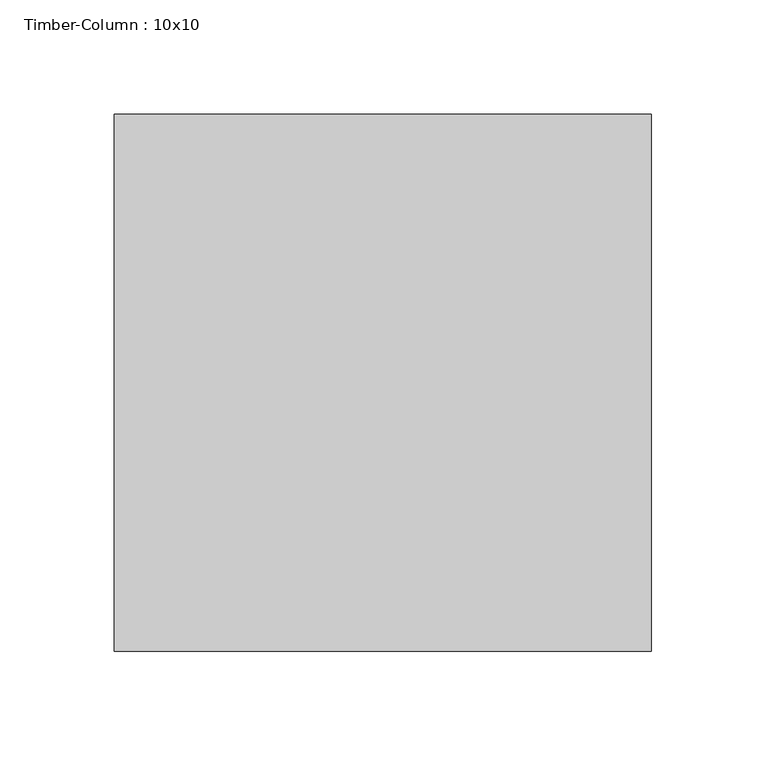
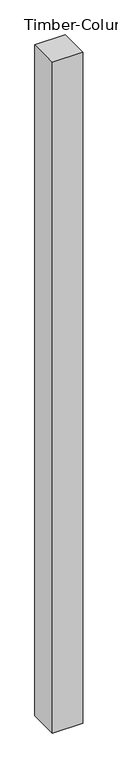
"""IFC4 building model written with IfcOpenShell, lengths in millimetres: column geometry, Timber-Column : 10x10."""

from ifc_helpers import new_model, si_unit, origin, origin_with_axes, place, context, project, spatial, polyline, outline, extrude, source, transform, mapped, element, save


def timber_column_10x10_5c3dec59(model_context):
    return source(origin(), model_context, "Body", "SweptSolid", [
        extrude(outline(polyline([(117.475, 117.475), (117.475, -117.475), (-117.475, -117.475), (-117.475, 117.475), (117.475, 117.475)])), origin_with_axes(), (0.0, 0.0, 1.0), 5486.4),
    ])


if __name__ == "__main__":
    model = new_model("IFC4")
    model_context = context("Model", 3, world=origin())
    ifc_project = project(units=[si_unit("LENGTHUNIT", "METRE", prefix="MILLI")], contexts=[model_context])
    site = spatial("IfcSite", under=ifc_project)
    building = spatial("IfcBuilding", under=site)
    placement = place(None, origin())
    timber_column_10x10_shape = timber_column_10x10_5c3dec59(model_context)
    element("IfcColumn", 1, ObjectType="Timber-Column : 10x10", at=placement, inside=building, context=model_context, shape_type="MappedRepresentation", body=[
        mapped(timber_column_10x10_shape, transform((0.0, 0.0, 0.0), x_axis=(1.0, 0.0, 0.0), y_axis=(0.0, 1.0, 0.0), z_axis=(0.0, 0.0, 1.0))),
    ])
    save(model, "model.ifc")

# Revit data of these elements
# Type "Timber-Column : 10x10"
#   Assembly Code = "B10"
#   A = 0.210069 SF
#   b = 0' - 9 1/4"
#   d = 0' - 9 1/4"
#   Structural Material = (4) CHARRED SISTERED 2X10s AT BEAM
# Element 1 (IfcColumn, "Timber-Column : 10x10")
#   Materials on its faces: "(4) CHARRED SISTERED 2X10s AT BEAM"
# Materials
#   "(4) CHARRED SISTERED 2X10s AT BEAM": class "Wood", colour RGB 144 144 144, transparency 0, Description = "Pinus Echinata", Cost = 0
